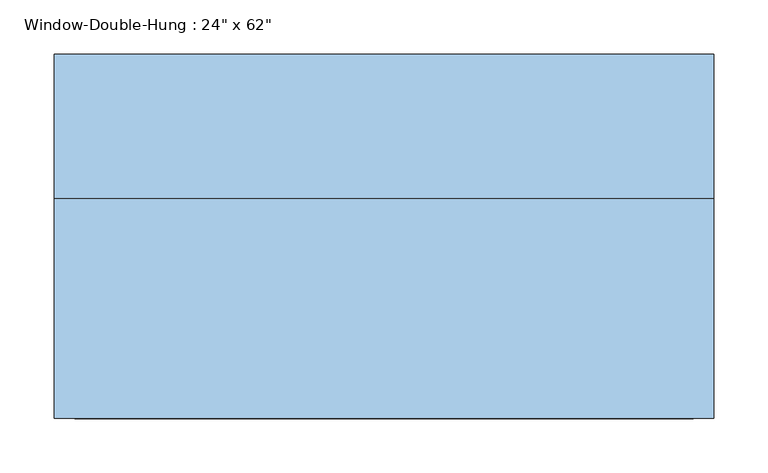
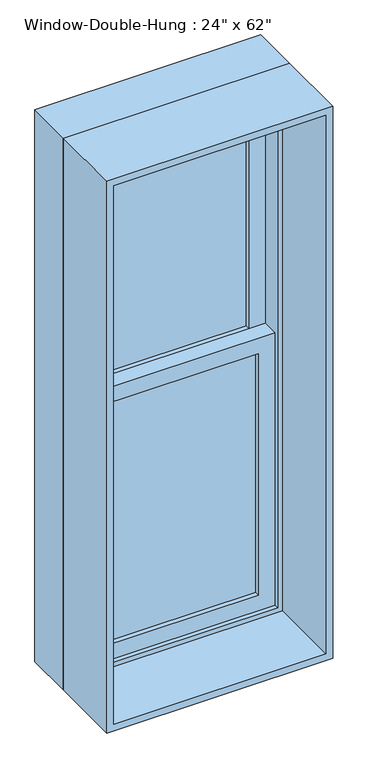
"""IFC4 building model written with IfcOpenShell, lengths in millimetres: window geometry."""

import ifcopenshell
import ifcopenshell.guid

model = None  # the IFC model being written
_history = None  # IfcOwnerHistory: only IFC2X3 demands one
_inside = {}  # id of a spatial element -> (the spatial element, [elements in it])
_under = {}  # id of a project, library or spatial element -> (it, [spatial elements below it])
_declared = {}  # id of a project -> (the project, [libraries it declares])
_typed = {}  # id of a type object -> (the type object, [elements of that type])
_made_of = {}  # id of a material, layer set ... -> (it, [elements and type objects made of it])


def new_model(schema):
    """Start an empty IFC model of exactly this schema.

    Asked for "IFC4X3", IfcOpenShell would pick the latest addendum, in which some entities
    have other attributes; the version numbers below select the first issue.
    IFC2X3 requires an IfcOwnerHistory on every rooted entity: one is made here for all.
    """
    global model, _history
    if schema == "IFC4X3":
        model = ifcopenshell.file(schema_version=(4, 3, 0, 0))
    else:
        model = ifcopenshell.file(schema=schema)
    _inside.clear()
    _under.clear()
    _declared.clear()
    _typed.clear()
    _made_of.clear()
    _history = None
    if model.schema == "IFC2X3":
        org = make("IfcOrganization", Name="unknown")
        user = make(
            "IfcPersonAndOrganization",
            ThePerson=make("IfcPerson", FamilyName="unknown"),
            TheOrganization=org,
        )
        app = make(
            "IfcApplication",
            ApplicationDeveloper=org,
            Version="unknown",
            ApplicationFullName="unknown",
            ApplicationIdentifier="unknown",
        )
        _history = make(
            "IfcOwnerHistory",
            OwningUser=user,
            OwningApplication=app,
            ChangeAction="ADDED",
            CreationDate=0,
        )
    return model


def make(cls, **values):
    """One entity of the class cls with the attributes given. An attribute that is None is left unset."""
    return model.create_entity(
        cls, **{name: value for name, value in values.items() if value is not None}
    )


def rooted(cls, **values):
    """An entity with a GlobalId (a new one), such as an element, a storey or a relation."""
    return make(cls, GlobalId=ifcopenshell.guid.new(), OwnerHistory=_history, **values)


def si_unit(unit_type, name, prefix=None):
    """IfcSIUnit, for example si_unit("LENGTHUNIT", "METRE", prefix="MILLI")."""
    return make("IfcSIUnit", UnitType=unit_type, Prefix=prefix, Name=name)


def assignment(units):
    """IfcUnitAssignment: the units of a project."""
    return None if units is None else make("IfcUnitAssignment", Units=units)


def point(xyz):
    """IfcCartesianPoint."""
    return None if xyz is None else make("IfcCartesianPoint", Coordinates=xyz)


def direction(xyz):
    """IfcDirection."""
    return None if xyz is None else make("IfcDirection", DirectionRatios=xyz)


def frame(location, z_axis=None, x_axis=None):
    """IfcAxis2Placement3D, a coordinate frame: its origin and axes. An axis left out is left unset."""
    return make(
        "IfcAxis2Placement3D",
        Location=point(location),
        Axis=direction(z_axis),
        RefDirection=direction(x_axis),
    )


def origin():
    """The frame at (0, 0, 0) with its axes left unset."""
    return frame((0.0, 0.0, 0.0))


def place(relative_to, where):
    """IfcLocalPlacement: puts the frame where relative to a parent placement (None: the world)."""
    return make(
        "IfcLocalPlacement", PlacementRelTo=relative_to, RelativePlacement=where
    )


def context(
    kind, dimensions, precision=None, world=None, true_north=None, identifier=None
):
    """IfcGeometricRepresentationContext, for example the 3D "Model" context."""
    return make(
        "IfcGeometricRepresentationContext",
        ContextIdentifier=identifier,
        ContextType=kind,
        CoordinateSpaceDimension=dimensions,
        Precision=precision,
        WorldCoordinateSystem=world,
        TrueNorth=true_north,
    )


def project(units=None, contexts=None):
    """IfcProject with its units and contexts."""
    return rooted(
        "IfcProject",
        Name="project",
        RepresentationContexts=contexts,
        UnitsInContext=assignment(units),
    )


def spatial(cls, under=None, at=None, **own):
    """A site, building, storey or space (cls), placed at a placement, below another one or the project."""
    s = rooted(cls, ObjectPlacement=at, **own)
    if under is not None:
        _under.setdefault(under.id(), (under, []))[1].append(s)
    return s


def polyline(points):
    """IfcPolyline through the points."""
    return make("IfcPolyline", Points=[point(p) for p in points])


def outline(outer, holes=None, kind="AREA"):
    """IfcArbitraryClosedProfileDef: a profile drawn as a closed curve; with holes, ...WithVoids."""
    if holes is None:
        return make("IfcArbitraryClosedProfileDef", ProfileType=kind, OuterCurve=outer)
    return make(
        "IfcArbitraryProfileDefWithVoids",
        ProfileType=kind,
        OuterCurve=outer,
        InnerCurves=holes,
    )


def extrude(swept, where, along, depth):
    """IfcExtrudedAreaSolid: the profile swept, set in the frame where, extruded along a direction by depth."""
    return make(
        "IfcExtrudedAreaSolid",
        SweptArea=swept,
        Position=where,
        ExtrudedDirection=direction(along),
        Depth=depth,
    )


def shape(context_of_items, identifier, shape_type, items):
    """IfcShapeRepresentation: the items that make up one representation, for example the "Body"."""
    return make(
        "IfcShapeRepresentation",
        ContextOfItems=context_of_items,
        RepresentationIdentifier=identifier,
        RepresentationType=shape_type,
        Items=items,
    )


def source(mapping_origin, context_of_items, identifier, shape_type, items):
    """IfcRepresentationMap: a shape defined once, which mapped items show again and again."""
    return make(
        "IfcRepresentationMap",
        MappingOrigin=mapping_origin,
        MappedRepresentation=shape(context_of_items, identifier, shape_type, items),
    )


def transform(
    local_origin,
    x_axis=None,
    y_axis=None,
    z_axis=None,
    scale=None,
    scale2=None,
    scale3=None,
    uniform=True,
):
    """IfcCartesianTransformationOperator3D, or its non-uniform kind. x_axis, y_axis, z_axis: its Axis1, 2, 3."""
    if uniform:
        return make(
            "IfcCartesianTransformationOperator3D",
            Axis1=direction(x_axis),
            Axis2=direction(y_axis),
            LocalOrigin=point(local_origin),
            Scale=scale,
            Axis3=direction(z_axis),
        )
    return make(
        "IfcCartesianTransformationOperator3DnonUniform",
        Axis1=direction(x_axis),
        Axis2=direction(y_axis),
        LocalOrigin=point(local_origin),
        Scale=scale,
        Axis3=direction(z_axis),
        Scale2=scale2,
        Scale3=scale3,
    )


def mapped(mapping_source, mapping_target):
    """IfcMappedItem: shows the shape of a source again, moved by a transform."""
    return make(
        "IfcMappedItem", MappingSource=mapping_source, MappingTarget=mapping_target
    )


def made_of(thing, what):
    """Note that an element or type object is made of a material, layer set ...; save() writes the relation."""
    if what is not None:
        _made_of.setdefault(what.id(), (what, []))[1].append(thing)
    return thing


def element(
    cls,
    number,
    at=None,
    inside=None,
    cuts=None,
    type_object=None,
    material=None,
    context=None,
    identifier="Body",
    shape_type=None,
    held_by="IfcProductDefinitionShape",
    body=None,
    shapes=None,
    **own,
):
    """One element of the class cls, such as IfcWall. Its Tag is "e" and its number.

    at: its placement. inside: the storey or other place that contains it. cuts: it is an
    opening in that element (IfcRelVoidsElement). A single representation is given by context,
    identifier, shape_type and body (its items); several are given by shapes. held_by: the class
    of the entity that holds the representations. save() writes the other relations.
    """
    e = rooted(cls, Tag="e%d" % number, ObjectPlacement=at, **own)
    if body is not None:
        shapes = [shape(context, identifier, shape_type, body)]
    if shapes is not None:
        e.Representation = make(held_by, Representations=shapes)
    if inside is not None:
        _inside.setdefault(inside.id(), (inside, []))[1].append(e)
    if cuts is not None:
        rooted(
            "IfcRelVoidsElement", RelatingBuildingElement=cuts, RelatedOpeningElement=e
        )
    if type_object is not None:
        _typed.setdefault(type_object.id(), (type_object, []))[1].append(e)
    return made_of(e, material)


def aggregate(whole, parts):
    """IfcRelAggregates: a whole, such as a stair, and the parts it consists of."""
    return rooted("IfcRelAggregates", RelatingObject=whole, RelatedObjects=parts)


def save(model, path):
    """Write the relations noted so far, then the file.

    IfcRelAggregates (storeys below a building ...), IfcRelContainedInSpatialStructure (elements
    in a storey), IfcRelDefinesByType, IfcRelAssociatesMaterial and IfcRelDeclares: one each for
    every whole, place, type object, material and project.
    """
    for whole, parts in _under.values():
        aggregate(whole, parts)
    for where, things in _inside.values():
        rooted(
            "IfcRelContainedInSpatialStructure",
            RelatedElements=things,
            RelatingStructure=where,
        )
    for kind, things in _typed.values():
        rooted("IfcRelDefinesByType", RelatedObjects=things, RelatingType=kind)
    for what, things in _made_of.values():
        rooted("IfcRelAssociatesMaterial", RelatedObjects=things, RelatingMaterial=what)
    for by, libraries in _declared.values():
        rooted("IfcRelDeclares", RelatingContext=by, RelatedDefinitions=libraries)
    model.write(path)


def window_aa90209f(model_context):
    return source(origin(), model_context, "Body", "SweptSolid", [
        extrude(outline(polyline([(228.6, 88.9), (228.6, 82.55), (-228.6, 82.55), (-228.6, 88.9), (228.6, 88.9)])), frame((0.0, 0.0, 990.6), z_axis=(0.0, 0.0, 1.0), x_axis=(1.0, 0.0, 0.0)), (0.0, 0.0, 1.0), 688.975),
        extrude(outline(polyline([(-228.6, 76.2), (228.6, 76.2), (228.6, 69.85), (-228.6, 69.85), (-228.6, 76.2)])), frame((0.0, 0.0, 990.6), z_axis=(0.0, 0.0, 1.0), x_axis=(1.0, 0.0, 0.0)), (0.0, 0.0, 1.0), 688.975),
        extrude(outline(polyline([(228.6, 133.35), (228.6, 127.0), (-228.6, 127.0), (-228.6, 133.35), (228.6, 133.35)])), frame((0.0, 0.0, 1724.025), z_axis=(0.0, 0.0, 1.0), x_axis=(1.0, 0.0, 0.0)), (0.0, 0.0, 1.0), 688.975),
        extrude(outline(polyline([(-228.6, 120.65), (228.6, 120.65), (228.6, 114.3), (-228.6, 114.3), (-228.6, 120.65)])), frame((0.0, 0.0, 1724.025), z_axis=(0.0, 0.0, 1.0), x_axis=(1.0, 0.0, 0.0)), (0.0, 0.0, 1.0), 688.975),
        extrude(outline(polyline([(1724.025, -273.05), (946.15, -273.05), (946.15, 273.05), (1724.025, 273.05), (1724.025, -273.05)]), holes=[polyline([(1679.575, 228.6), (990.6, 228.6), (990.6, -228.6), (1679.575, -228.6), (1679.575, 228.6)])]), frame((0.0, 57.15, 0.0), z_axis=(0.0, 1.0, 0.0), x_axis=(0.0, 0.0, 1.0)), (0.0, 0.0, 1.0), 44.45),
        extrude(outline(polyline([(2457.45, -273.05), (1679.575, -273.05), (1679.575, 273.05), (2457.45, 273.05), (2457.45, -273.05)]), holes=[polyline([(2413.0, 228.6), (1724.025, 228.6), (1724.025, -228.6), (2413.0, -228.6), (2413.0, 228.6)])]), frame((0.0, 101.6, 0.0), z_axis=(0.0, 1.0, 0.0), x_axis=(0.0, 0.0, 1.0)), (0.0, 0.0, 1.0), 44.45),
        extrude(outline(polyline([(2489.2, -304.8), (914.4, -304.8), (914.4, 304.8), (2489.2, 304.8), (2489.2, -304.8)]), holes=[polyline([(2457.45, 273.05), (946.15, 273.05), (946.15, -273.05), (2457.45, -273.05), (2457.45, 273.05)])]), frame((0.0, 44.45, 0.0), z_axis=(0.0, 1.0, 0.0), x_axis=(0.0, 0.0, 1.0)), (0.0, 0.0, 1.0), 133.35),
        extrude(outline(polyline([(2489.2, 304.8), (2489.2, -304.8), (914.4, -304.8), (914.4, 304.8), (2489.2, 304.8)]), holes=[polyline([(2470.15, 285.75), (933.45, 285.75), (933.45, -285.75), (2470.15, -285.75), (2470.15, 285.75)])]), frame((0.0, -158.75, 0.0), z_axis=(0.0, 1.0, 0.0), x_axis=(0.0, 0.0, 1.0)), (0.0, 0.0, 1.0), 203.2),
    ])


if __name__ == "__main__":
    model = new_model("IFC4")
    model_context = context("Model", 3, world=origin())
    ifc_project = project(units=[si_unit("LENGTHUNIT", "METRE", prefix="MILLI")], contexts=[model_context])
    site = spatial("IfcSite", under=ifc_project)
    building = spatial("IfcBuilding", under=site)
    placement = place(None, origin())
    window_shape = window_aa90209f(model_context)
    element("IfcWindow", 1, ObjectType="Window-Double-Hung : 24\" x 62\"", at=placement, inside=building, context=model_context, shape_type="MappedRepresentation", body=[
        mapped(window_shape, transform((0.0, 0.0, 0.0), x_axis=(1.0, 0.0, 0.0), y_axis=(0.0, 1.0, 0.0), z_axis=(0.0, 0.0, 1.0))),
    ])
    save(model, "model.ifc")

# Revit data of these elements
# Type "Window-Double-Hung : 24\" x 62\""
#   Type Mark = "30"
#   Fire Rating = "0.5h"
#   Construction Type Id = "DG-DR"
#   Assembly Code = "B2020100"
#   Analytic Construction = "Double glazing - domestic"
#   Wall Thickness [instance default] = 0' - 6"
#   Window Inset [instance default] = 0' - 0"
#   Visual Light Transmittance = 0.81
#   Thermal Resistance (R) = 1.8146 (h·ft²·°F)/BTU
#   Solar Heat Gain Coefficient = 0.76
#   Muntin Width = 1' - 6"
#   Muntin Height = 2' - 3 1/8"
#   Interior Wall Closure [instance default] = 0' - 1 1/2"
#   Rough Width = 2' - 0 1/2"
#   Rough Height = 5' - 2 1/2"
#   Frame Extension [instance default] = 0' - 1 1/4"
#   Exterior Wall Closure [instance default] = 0' - 0 1/2"
#   Extension Jamb [instance default] = 0' - 1 1/2"
#   Heat Transfer Coefficient (U) = 0.5511 BTU/(h·ft²·°F)
#   Height = 5' - 2"
#   Width = 2' - 0"
#   Top Muntin Visibility = yes
#   Indicator Visibility [instance default] = yes
#   Extension Jamb Visibility [instance default] = yes
#   Interior Trim Visibility [instance default] = yes
#   Exterior Trim Visibility [instance default] = yes
#   Define Thermal Properties by = 1
#   Bottom Muntin Visibility = yes
#   Muntin Pattern = Muntin Pattern_2x2 : Muntin Pattern_2x2
#   Interior Trim Material = Wood - Stained
#   Interior Trim = Trim-Window-Interior-Flat : Picture Frame
#   Exterior Trim Material = Clad - White
#   Exterior Trim = Trim-Window-Exterior-Flat : with Sill
#   Glass Panel Material = Glass
#   Exterior Frame Material = Clad - White
#   Interior Frame Material = Wood - Stained
#   Wall Closure = (empty or 0)
# Element 1 (IfcWindow, "Window-Double-Hung : 24\" x 62\"")
#   Wall Thickness = 1' - 0 1/2"
#   Extension Jamb = 0' - 8"
#   Materials on its faces: "Wood - Stained", "Glass", "Clad - White"
# Materials
#   "Wood - Stained": class "Wood", colour RGB 224 178 126, transparency 0, Cost = 0
#   "Clad - White": class "Wood", colour RGB 245 245 243, transparency 0, Cost = 0
#   "Glass": class "Glass", colour RGB 0 128 192, transparency 0.75, Description = "Soda Lime Glass", Cost = 0
